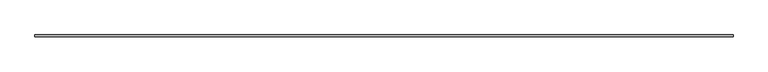
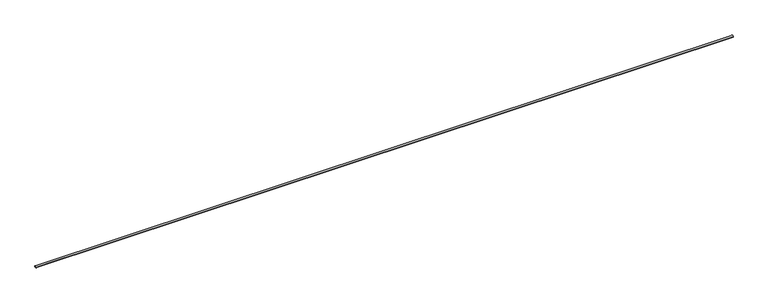
"""IFC4 building model written with IfcOpenShell, lengths in millimetres: proxy geometry, TN_Проводник с держателем_Молниезащита : Проводник 8 мм с держателем провода-молниеотвода 75х130 пустой (50 шт/уп)."""

from ifc_helpers import new_model, si_unit, point, frame, frame_2d, origin, place, context, project, spatial, circle_curve, trimmed, segment, composite_curve, outline, extrude, source, transform, mapped, element, save


def specialty_equipment_f2b8546d(model_context):
    return source(origin(), model_context, "Body", "SweptSolid", [
        extrude(outline(composite_curve([segment(trimmed(circle_curve(frame_2d((0.0, 69.0)), 3.9911911), [point((-3.9911911, 69.0))], [point((3.9911911, 69.0))], False, "CARTESIAN"), True, "CONTINUOUS"), segment(trimmed(circle_curve(frame_2d((0.0, 69.0)), 3.9911911), [point((3.9911911, 69.0))], [point((-3.9911911, 69.0))], False, "CARTESIAN"), True, "CONTINUOUS")], self_intersect=False)), frame((-100.0, 0.0, 0.0), z_axis=(1.0, 0.0, 0.0), x_axis=(0.0, 1.0, 0.0)), (0.0, 0.0, 1.0), 3000.0),
    ])


if __name__ == "__main__":
    model = new_model("IFC4")
    model_context = context("Model", 3, world=origin())
    ifc_project = project(units=[si_unit("LENGTHUNIT", "METRE", prefix="MILLI")], contexts=[model_context])
    site = spatial("IfcSite", under=ifc_project)
    building = spatial("IfcBuilding", under=site)
    placement = place(None, origin())
    specialty_equipment_shape = specialty_equipment_f2b8546d(model_context)
    element("IfcBuildingElementProxy", 1, Name="TN_Проводник с держателем_Молниезащита : Проводник 8 мм с держателем провода-молниеотвода 75х130 пустой (50 шт/уп)", ObjectType="TN_Проводник с держателем_Молниезащита : Проводник 8 мм с держателем провода-молниеотвода 75х130 пустой (50 шт/уп)", at=placement, inside=building, context=model_context, shape_type="MappedRepresentation", body=[
        mapped(specialty_equipment_shape, transform((0.0, 0.0, 0.0), x_axis=(1.0, 0.0, 0.0), y_axis=(0.0, 1.0, 0.0), z_axis=(0.0, 0.0, 1.0))),
    ])
    save(model, "model.ifc")

# Revit data of these elements
# Type "TN_Проводник с держателем_Молниезащита : Проводник 8 мм с держателем провода-молниеотвода 75х130 пустой (50 шт/уп)"
#   Description = "Проводник для молниеотвода"
#   Type Comments = "п.м."
#   Manufacturer = "ТехноНИКОЛЬ"
#   ADSK_Примечание = ""
#   ADSK_Обозначение [instance default] = "ТехноНИКОЛЬ"
#   ADSK_Наименование = "Проводник 8мм"
#   ADSK_Масса_Текст = ""
#   ADSK_Марка = ""
#   ADSK_Код изделия = ""
#   ADSK_Завод-изготовитель [instance default] = "ТехноНИКОЛЬ"
#   ADSK_Единица измерения [instance default] = "п.м."
#   ADSK_Группирование = "Комплектующие и воронки"
#   ADSK_URL страницы изделия = ""
#   ADSK_URL документации изделия = ""
#   built-in parameter 1001306 [instance default] = 10.7243 (stored number, unit not read)
#   Выступ проводника справа [instance default] = 100 mm
#   Выступ проводника слева [instance default] = 100 mm
#   ADSK_Размер_Длина [instance default] = 3468.767 mm
#   ADSK_Количество [instance default] = 3.46877
#   Количество держателей [instance default] = 3
#   ADSK_Материал = TN_СтальГальванизированная_Серый
#   Default Elevation = 0
#   URL = ""
# Element 1 (IfcBuildingElementProxy, "TN_Проводник с держателем_Молниезащита : Проводник 8 мм с держателем провода-молниеотвода 75х130 пустой (50 шт/уп)")
#   built-in parameter 1001306 = 9.18635 (stored number, unit not read)
#   ADSK_Размер_Длина = 3000 mm
#   ADSK_Количество = 3
#   Materials on its faces: "TN_СтальГальванизированная_Серый"
# Materials
#   "TN_СтальГальванизированная_Серый": class "Типовые", colour RGB 206 210 213, transparency 0, Cost = 0
